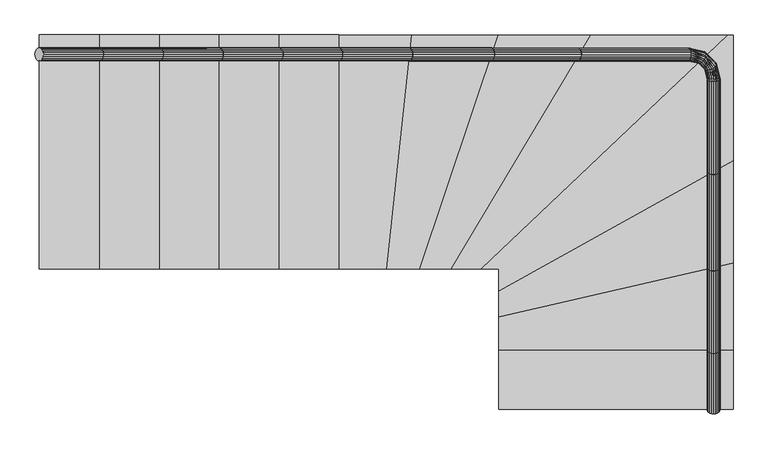
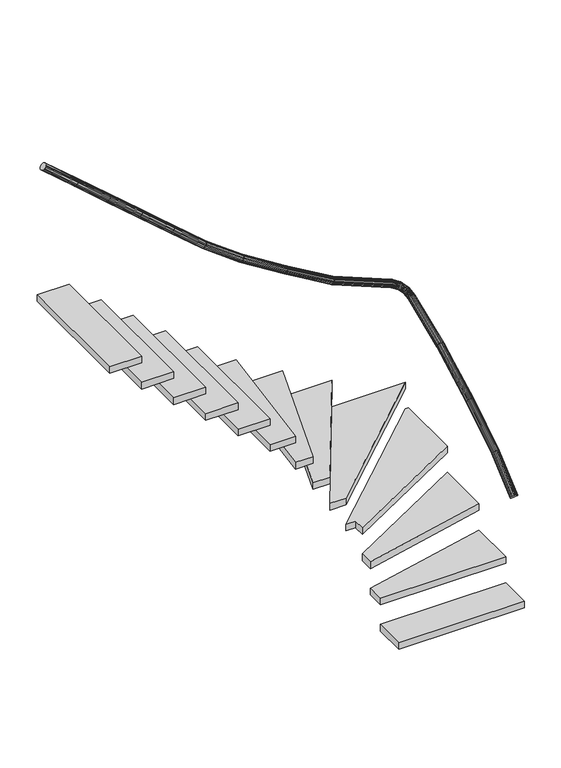
"""IFC4 building model written with IfcOpenShell, lengths in millimetres: stair geometry, 0_3d."""

import ifcopenshell
import ifcopenshell.guid

model = None  # the IFC model being written
_history = None  # IfcOwnerHistory: only IFC2X3 demands one
_inside = {}  # id of a spatial element -> (the spatial element, [elements in it])
_under = {}  # id of a project, library or spatial element -> (it, [spatial elements below it])
_declared = {}  # id of a project -> (the project, [libraries it declares])
_typed = {}  # id of a type object -> (the type object, [elements of that type])
_made_of = {}  # id of a material, layer set ... -> (it, [elements and type objects made of it])


def new_model(schema):
    """Start an empty IFC model of exactly this schema.

    Asked for "IFC4X3", IfcOpenShell would pick the latest addendum, in which some entities
    have other attributes; the version numbers below select the first issue.
    IFC2X3 requires an IfcOwnerHistory on every rooted entity: one is made here for all.
    """
    global model, _history
    if schema == "IFC4X3":
        model = ifcopenshell.file(schema_version=(4, 3, 0, 0))
    else:
        model = ifcopenshell.file(schema=schema)
    _inside.clear()
    _under.clear()
    _declared.clear()
    _typed.clear()
    _made_of.clear()
    _history = None
    if model.schema == "IFC2X3":
        org = make("IfcOrganization", Name="unknown")
        user = make(
            "IfcPersonAndOrganization",
            ThePerson=make("IfcPerson", FamilyName="unknown"),
            TheOrganization=org,
        )
        app = make(
            "IfcApplication",
            ApplicationDeveloper=org,
            Version="unknown",
            ApplicationFullName="unknown",
            ApplicationIdentifier="unknown",
        )
        _history = make(
            "IfcOwnerHistory",
            OwningUser=user,
            OwningApplication=app,
            ChangeAction="ADDED",
            CreationDate=0,
        )
    return model


def make(cls, **values):
    """One entity of the class cls with the attributes given. An attribute that is None is left unset."""
    return model.create_entity(
        cls, **{name: value for name, value in values.items() if value is not None}
    )


def rooted(cls, **values):
    """An entity with a GlobalId (a new one), such as an element, a storey or a relation."""
    return make(cls, GlobalId=ifcopenshell.guid.new(), OwnerHistory=_history, **values)


def si_unit(unit_type, name, prefix=None):
    """IfcSIUnit, for example si_unit("LENGTHUNIT", "METRE", prefix="MILLI")."""
    return make("IfcSIUnit", UnitType=unit_type, Prefix=prefix, Name=name)


def assignment(units):
    """IfcUnitAssignment: the units of a project."""
    return None if units is None else make("IfcUnitAssignment", Units=units)


def point(xyz):
    """IfcCartesianPoint."""
    return None if xyz is None else make("IfcCartesianPoint", Coordinates=xyz)


def direction(xyz):
    """IfcDirection."""
    return None if xyz is None else make("IfcDirection", DirectionRatios=xyz)


def frame(location, z_axis=None, x_axis=None):
    """IfcAxis2Placement3D, a coordinate frame: its origin and axes. An axis left out is left unset."""
    return make(
        "IfcAxis2Placement3D",
        Location=point(location),
        Axis=direction(z_axis),
        RefDirection=direction(x_axis),
    )


def origin():
    """The frame at (0, 0, 0) with its axes left unset."""
    return frame((0.0, 0.0, 0.0))


def origin_with_axes():
    """The frame at (0, 0, 0) with the z axis (0, 0, 1) and the x axis (1, 0, 0) written out."""
    return frame((0.0, 0.0, 0.0), z_axis=(0.0, 0.0, 1.0), x_axis=(1.0, 0.0, 0.0))


def place(relative_to, where):
    """IfcLocalPlacement: puts the frame where relative to a parent placement (None: the world)."""
    return make(
        "IfcLocalPlacement", PlacementRelTo=relative_to, RelativePlacement=where
    )


def context(
    kind, dimensions, precision=None, world=None, true_north=None, identifier=None
):
    """IfcGeometricRepresentationContext, for example the 3D "Model" context."""
    return make(
        "IfcGeometricRepresentationContext",
        ContextIdentifier=identifier,
        ContextType=kind,
        CoordinateSpaceDimension=dimensions,
        Precision=precision,
        WorldCoordinateSystem=world,
        TrueNorth=true_north,
    )


def project(units=None, contexts=None):
    """IfcProject with its units and contexts."""
    return rooted(
        "IfcProject",
        Name="project",
        RepresentationContexts=contexts,
        UnitsInContext=assignment(units),
    )


def spatial(cls, under=None, at=None, **own):
    """A site, building, storey or space (cls), placed at a placement, below another one or the project."""
    s = rooted(cls, ObjectPlacement=at, **own)
    if under is not None:
        _under.setdefault(under.id(), (under, []))[1].append(s)
    return s


def polyline(points):
    """IfcPolyline through the points."""
    return make("IfcPolyline", Points=[point(p) for p in points])


def outline(outer, holes=None, kind="AREA"):
    """IfcArbitraryClosedProfileDef: a profile drawn as a closed curve; with holes, ...WithVoids."""
    if holes is None:
        return make("IfcArbitraryClosedProfileDef", ProfileType=kind, OuterCurve=outer)
    return make(
        "IfcArbitraryProfileDefWithVoids",
        ProfileType=kind,
        OuterCurve=outer,
        InnerCurves=holes,
    )


def extrude(swept, where, along, depth):
    """IfcExtrudedAreaSolid: the profile swept, set in the frame where, extruded along a direction by depth."""
    return make(
        "IfcExtrudedAreaSolid",
        SweptArea=swept,
        Position=where,
        ExtrudedDirection=direction(along),
        Depth=depth,
    )


def faces_of(points, faces, orient=None, outer=None):
    """IfcFace entities. A face is a list of loops; a loop is a list of indices into points, from 0.

    orient and outer hold one flag for each loop. By default every Orientation is true, the
    first loop of a face is its IfcFaceOuterBound and the others are IfcFaceBound.
    """
    made = []
    for i, loops in enumerate(faces):
        bounds = []
        for j, loop in enumerate(loops):
            is_outer = j == 0 if outer is None else outer[i][j]
            bounds.append(
                make(
                    "IfcFaceOuterBound" if is_outer else "IfcFaceBound",
                    Bound=make("IfcPolyLoop", Polygon=[points[k] for k in loop]),
                    Orientation=True if orient is None else orient[i][j],
                )
            )
        made.append(make("IfcFace", Bounds=bounds))
    return made


def faceted_brep(points, faces, orient=None, outer=None, voids=None):
    """IfcFacetedBrep: a solid bounded by flat faces; with voids (closed shells), ...WithVoids."""
    shared = [point(p) for p in points]
    hull = make("IfcClosedShell", CfsFaces=faces_of(shared, faces, orient, outer))
    if voids is None:
        return make("IfcFacetedBrep", Outer=hull)
    return make(
        "IfcFacetedBrepWithVoids",
        Outer=hull,
        Voids=[
            make(cls, CfsFaces=faces_of(shared, fs, o, b)) for cls, fs, o, b in voids
        ],
    )


def shape(context_of_items, identifier, shape_type, items):
    """IfcShapeRepresentation: the items that make up one representation, for example the "Body"."""
    return make(
        "IfcShapeRepresentation",
        ContextOfItems=context_of_items,
        RepresentationIdentifier=identifier,
        RepresentationType=shape_type,
        Items=items,
    )


def source(mapping_origin, context_of_items, identifier, shape_type, items):
    """IfcRepresentationMap: a shape defined once, which mapped items show again and again."""
    return make(
        "IfcRepresentationMap",
        MappingOrigin=mapping_origin,
        MappedRepresentation=shape(context_of_items, identifier, shape_type, items),
    )


def transform(
    local_origin,
    x_axis=None,
    y_axis=None,
    z_axis=None,
    scale=None,
    scale2=None,
    scale3=None,
    uniform=True,
):
    """IfcCartesianTransformationOperator3D, or its non-uniform kind. x_axis, y_axis, z_axis: its Axis1, 2, 3."""
    if uniform:
        return make(
            "IfcCartesianTransformationOperator3D",
            Axis1=direction(x_axis),
            Axis2=direction(y_axis),
            LocalOrigin=point(local_origin),
            Scale=scale,
            Axis3=direction(z_axis),
        )
    return make(
        "IfcCartesianTransformationOperator3DnonUniform",
        Axis1=direction(x_axis),
        Axis2=direction(y_axis),
        LocalOrigin=point(local_origin),
        Scale=scale,
        Axis3=direction(z_axis),
        Scale2=scale2,
        Scale3=scale3,
    )


def mapped(mapping_source, mapping_target):
    """IfcMappedItem: shows the shape of a source again, moved by a transform."""
    return make(
        "IfcMappedItem", MappingSource=mapping_source, MappingTarget=mapping_target
    )


def made_of(thing, what):
    """Note that an element or type object is made of a material, layer set ...; save() writes the relation."""
    if what is not None:
        _made_of.setdefault(what.id(), (what, []))[1].append(thing)
    return thing


def element(
    cls,
    number,
    at=None,
    inside=None,
    cuts=None,
    type_object=None,
    material=None,
    context=None,
    identifier="Body",
    shape_type=None,
    held_by="IfcProductDefinitionShape",
    body=None,
    shapes=None,
    **own,
):
    """One element of the class cls, such as IfcWall. Its Tag is "e" and its number.

    at: its placement. inside: the storey or other place that contains it. cuts: it is an
    opening in that element (IfcRelVoidsElement). A single representation is given by context,
    identifier, shape_type and body (its items); several are given by shapes. held_by: the class
    of the entity that holds the representations. save() writes the other relations.
    """
    e = rooted(cls, Tag="e%d" % number, ObjectPlacement=at, **own)
    if body is not None:
        shapes = [shape(context, identifier, shape_type, body)]
    if shapes is not None:
        e.Representation = make(held_by, Representations=shapes)
    if inside is not None:
        _inside.setdefault(inside.id(), (inside, []))[1].append(e)
    if cuts is not None:
        rooted(
            "IfcRelVoidsElement", RelatingBuildingElement=cuts, RelatedOpeningElement=e
        )
    if type_object is not None:
        _typed.setdefault(type_object.id(), (type_object, []))[1].append(e)
    return made_of(e, material)


def aggregate(whole, parts):
    """IfcRelAggregates: a whole, such as a stair, and the parts it consists of."""
    return rooted("IfcRelAggregates", RelatingObject=whole, RelatedObjects=parts)


def save(model, path):
    """Write the relations noted so far, then the file.

    IfcRelAggregates (storeys below a building ...), IfcRelContainedInSpatialStructure (elements
    in a storey), IfcRelDefinesByType, IfcRelAssociatesMaterial and IfcRelDeclares: one each for
    every whole, place, type object, material and project.
    """
    for whole, parts in _under.values():
        aggregate(whole, parts)
    for where, things in _inside.values():
        rooted(
            "IfcRelContainedInSpatialStructure",
            RelatedElements=things,
            RelatingStructure=where,
        )
    for kind, things in _typed.values():
        rooted("IfcRelDefinesByType", RelatedObjects=things, RelatingType=kind)
    for what, things in _made_of.values():
        rooted("IfcRelAssociatesMaterial", RelatedObjects=things, RelatingMaterial=what)
    for by, libraries in _declared.values():
        rooted("IfcRelDeclares", RelatingContext=by, RelatedDefinitions=libraries)
    model.write(path)


def stair_9e6d9002(model_context):
    return source(origin(), model_context, "Body", "SolidModel", [
        extrude(outline(polyline([(1781.5036957, 473.824936), (1781.5036957, 556.9018591), (1711.5036957, 556.9018591), (2658.8332796, 1456.9018591), (2681.5036957, 1456.9018591), (2681.5036957, 973.1970565), (1781.5036957, 473.824936)])), frame((0.0, 0.0, 595.7142857), z_axis=(0.0, 0.0, 1.0), x_axis=(1.0, 0.0, 0.0)), (0.0, 0.0, 1.0), 50.0),
        extrude(outline(polyline([(936.9018591, 556.9018591), (706.9018591, 556.9018591), (706.9018591, 1456.9018591), (936.9018591, 1456.9018591), (936.9018591, 556.9018591)])), frame((0.0, 0.0, 1787.1428571), z_axis=(0.0, 0.0, 1.0), x_axis=(1.0, 0.0, 0.0)), (0.0, 0.0, 1.0), 50.0),
        extrude(outline(polyline([(1.2235871, -7.9923214), (0.0, 0.0), (1.2235871, 7.9923214), (4.7745751, 15.2022987), (10.3053687, 20.9241691), (17.2745751, 24.597836), (25.0, 25.8636953), (32.7254248, 24.597836), (39.6946313, 20.9241691), (45.2254248, 15.2022987), (48.7764129, 7.9923214), (50.0, 0.0), (48.7764129, -7.9923214), (45.2254248, -15.2022986), (39.6946313, -20.9241689), (32.7254248, -24.5978359), (25.0, -25.8636953), (17.2745751, -24.5978359), (10.3053687, -20.9241689), (4.7745751, -15.2022986), (1.2235871, -7.9923214)])), frame((936.9018591, 1406.9018591, 2656.7020937), z_axis=(-0.7569287102857389, 0.0, 0.6534974579485127), x_axis=(0.0, -1.0, 0.0)), (0.0, 0.0, 1.0), 303.8595272),
        extrude(outline(polyline([(1349.1921789, 556.9018591), (1166.9018591, 556.9018591), (1166.9018591, 1456.9018591), (1444.6115394, 1456.9018591), (1349.1921789, 556.9018591)])), frame((0.0, 0.0, 1390.0), z_axis=(0.0, 0.0, 1.0), x_axis=(1.0, 0.0, 0.0)), (0.0, 0.0, 1.0), 50.0),
        extrude(outline(polyline([(1477.0220692, 556.9018591), (1349.1921789, 556.9018591), (1444.6115394, 1456.9018591), (1776.781649, 1456.9018591), (1477.0220692, 556.9018591)])), frame((0.0, 0.0, 1191.4285714), z_axis=(0.0, 0.0, 1.0), x_axis=(1.0, 0.0, 0.0)), (0.0, 0.0, 1.0), 50.0),
        extrude(outline(polyline([(1711.5036957, 556.9018591), (1597.1723093, 556.9018591), (2132.6233472, 1456.9018591), (2658.8332796, 1456.9018591), (1711.5036957, 556.9018591)])), frame((0.0, 0.0, 794.2857143), z_axis=(0.0, 0.0, 1.0), x_axis=(1.0, 0.0, 0.0)), (0.0, 0.0, 1.0), 50.0),
        extrude(outline(polyline([(1.2235871, -7.9923214), (0.0, 0.0), (1.2235871, 7.9923214), (4.7745751, 15.2022986), (10.3053687, 20.924169), (17.2745751, 24.5978359), (25.0, 25.8636953), (32.7254248, 24.5978359), (39.6946313, 20.924169), (45.2254248, 15.2022986), (48.7764129, 7.9923214), (50.0, 0.0), (48.7764129, -7.9923214), (45.2254248, -15.2022986), (39.6946313, -20.924169), (32.7254248, -24.597836), (25.0, -25.8636953), (17.2745751, -24.597836), (10.3053687, -20.924169), (4.7745751, -15.2022986), (1.2235871, -7.9923214)])), frame((246.9018591, 1406.9018591, 3252.4163795), z_axis=(-0.7569287102857456, 0.0, 0.6534974579485049), x_axis=(0.0, -1.0, 0.0)), (0.0, 0.0, 1.0), 303.8595272),
        faceted_brep([(2630.2801086, 935.0213576, 1458.0478269), (2631.5036957, 931.5827131, 1465.2735223), (2630.2801086, 928.1440687, 1472.4992177), (2626.7291206, 925.0420228, 1479.0176117), (2621.198327, 922.5802252, 1484.1906384), (2614.2291206, 920.9996538, 1487.511926), (2606.5036957, 920.4550261, 1488.6563638), (2598.7782709, 920.9996538, 1487.511926), (2591.8090644, 922.5802252, 1484.1906384), (2586.2782709, 925.0420228, 1479.0176117), (2582.7272828, 928.1440687, 1472.4992177), (2581.5036957, 931.5827131, 1465.2735223), (2582.7272828, 935.0213576, 1458.0478269), (2586.2782709, 938.1234035, 1451.529433), (2591.8090644, 940.5852011, 1446.3564062), (2598.7782709, 942.1657724, 1443.0351186), (2606.5036957, 942.7104002, 1441.8906809), (2614.2291206, 942.1657724, 1443.0351186), (2621.198327, 940.5852011, 1446.3564062), (2626.7291206, 938.1234035, 1451.529433), (2630.2801086, 1283.3224302, 1620.3777918), (2631.5036957, 1286.3944101, 1612.9994356), (2630.2801086, 1289.46639, 1605.6210794), (2626.7291206, 1292.2376632, 1598.9649681), (2621.198327, 1294.436958, 1593.6826483), (2614.2291206, 1295.8489921, 1590.2911902), (2606.5036957, 1296.335546, 1589.1225734), (2598.7782709, 1295.8489921, 1590.2911902), (2591.8090644, 1294.436958, 1593.6826483), (2586.2782709, 1292.2376632, 1598.9649681), (2582.7272828, 1289.46639, 1605.6210794), (2581.5036957, 1286.3944101, 1612.9994356), (2582.7272828, 1283.3224302, 1620.3777918), (2586.2782709, 1280.5511571, 1627.0339031), (2591.8090644, 1278.3518623, 1632.3162229), (2598.7782709, 1276.9398281, 1635.707681), (2606.5036957, 1276.4532743, 1636.8762979), (2614.2291206, 1276.9398281, 1635.707681), (2621.198327, 1278.3518623, 1632.3162229), (2626.7291206, 1280.5511571, 1627.0339031)], [[[0, 1, 2, 3, 4, 5, 6, 7, 8, 9, 10, 11, 12, 13, 14, 15, 16, 17, 18, 19]], [[20, 21, 22, 23, 24, 25, 26, 27, 28, 29, 30, 31, 32, 33, 34, 35, 36, 37, 38, 39]], [[2, 1, 21, 20]], [[3, 2, 20, 39]], [[4, 3, 39, 38]], [[5, 4, 38, 37]], [[6, 5, 37, 36]], [[7, 6, 36, 35]], [[8, 7, 35, 34]], [[9, 8, 34, 33]], [[10, 9, 33, 32]], [[11, 10, 32, 31]], [[12, 11, 31, 30]], [[13, 12, 30, 29]], [[14, 13, 29, 28]], [[15, 14, 28, 27]], [[16, 15, 27, 26]], [[17, 16, 26, 25]], [[18, 17, 25, 24]], [[19, 18, 24, 23]], [[0, 19, 23, 22]], [[1, 0, 22, 21]]]),
        extrude(outline(polyline([(1781.5036957, 373.9346688), (1781.5036957, 473.824936), (2681.5036957, 973.1970565), (2681.5036957, 579.8690495), (1781.5036957, 373.9346688)])), frame((0.0, 0.0, 397.1428571), z_axis=(0.0, 0.0, 1.0), x_axis=(1.0, 0.0, 0.0)), (0.0, 0.0, 1.0), 50.0),
        extrude(outline(polyline([(1.2235871, -7.9923214), (0.0, 0.0), (1.2235871, 7.9923214), (4.7745751, 15.2022986), (10.3053687, 20.9241691), (17.2745751, 24.5978359), (25.0, 25.8636953), (32.7254248, 24.5978359), (39.6946313, 20.9241691), (45.2254248, 15.2022986), (48.7764129, 7.9923214), (50.0, 0.0), (48.7764129, -7.9923214), (45.2254248, -15.2022986), (39.6946313, -20.924169), (32.7254248, -24.5978359), (25.0, -25.8636953), (17.2745751, -24.5978359), (10.3053687, -20.924169), (4.7745751, -15.2022986), (1.2235871, -7.9923214)])), frame((476.9018591, 1406.9018591, 3053.8449509), z_axis=(-0.7569287102857636, 0.0, 0.6534974579484839), x_axis=(0.0, -1.0, 0.0)), (0.0, 0.0, 1.0), 303.8595272),
        faceted_brep([(2630.2801086, 566.7337566, 1259.7925307), (2631.5036957, 562.7078511, 1266.7020937), (2630.2801086, 558.6819455, 1273.6116568), (2626.7291206, 555.0501237, 1279.8448636), (2621.198327, 552.1678935, 1284.7915646), (2614.2291206, 550.3173878, 1287.9675421), (2606.5036957, 549.679747, 1289.0619094), (2598.7782709, 550.3173878, 1287.9675421), (2591.8090644, 552.1678935, 1284.7915646), (2586.2782709, 555.0501237, 1279.8448636), (2582.7272828, 558.6819455, 1273.6116568), (2581.5036957, 562.7078511, 1266.7020937), (2582.7272828, 566.7337566, 1259.7925307), (2586.2782709, 570.3655785, 1253.5593239), (2591.8090644, 573.2478087, 1248.6126229), (2598.7782709, 575.0983143, 1245.4366454), (2606.5036957, 575.7359551, 1244.3422781), (2614.2291206, 575.0983143, 1245.4366454), (2621.198327, 573.2478087, 1248.6126229), (2626.7291206, 570.3655785, 1253.5593239), (2630.2801086, 928.1440687, 1472.4992177), (2631.5036957, 931.5827131, 1465.2735223), (2630.2801086, 935.0213576, 1458.0478269), (2626.7291206, 938.1234035, 1451.529433), (2621.198327, 940.5852011, 1446.3564062), (2614.2291206, 942.1657724, 1443.0351186), (2606.5036957, 942.7104002, 1441.8906809), (2598.7782709, 942.1657724, 1443.0351186), (2591.8090644, 940.5852011, 1446.3564062), (2586.2782709, 938.1234035, 1451.529433), (2582.7272828, 935.0213576, 1458.0478269), (2581.5036957, 931.5827131, 1465.2735223), (2582.7272828, 928.1440687, 1472.4992177), (2586.2782709, 925.0420228, 1479.0176117), (2591.8090644, 922.5802252, 1484.1906384), (2598.7782709, 920.9996538, 1487.511926), (2606.5036957, 920.4550261, 1488.6563638), (2614.2291206, 920.9996538, 1487.511926), (2621.198327, 922.5802252, 1484.1906384), (2626.7291206, 925.0420228, 1479.0176117)], [[[0, 1, 2, 3, 4, 5, 6, 7, 8, 9, 10, 11, 12, 13, 14, 15, 16, 17, 18, 19]], [[20, 21, 22, 23, 24, 25, 26, 27, 28, 29, 30, 31, 32, 33, 34, 35, 36, 37, 38, 39]], [[2, 1, 21, 20]], [[3, 2, 20, 39]], [[4, 3, 39, 38]], [[5, 4, 38, 37]], [[6, 5, 37, 36]], [[7, 6, 36, 35]], [[8, 7, 35, 34]], [[9, 8, 34, 33]], [[10, 9, 33, 32]], [[11, 10, 32, 31]], [[12, 11, 31, 30]], [[13, 12, 30, 29]], [[14, 13, 29, 28]], [[15, 14, 28, 27]], [[16, 15, 27, 26]], [[17, 16, 26, 25]], [[18, 17, 25, 24]], [[19, 18, 24, 23]], [[0, 19, 23, 22]], [[1, 0, 22, 21]]]),
        faceted_brep([(2630.2801086, 251.6675536, 1061.6862641), (2631.5036957, 246.9018591, 1068.1306652), (2630.2801086, 242.1361647, 1074.5750662), (2626.7291206, 237.8369696, 1080.3886444), (2621.198327, 234.4251091, 1085.0023262), (2614.2291206, 232.2345598, 1087.9644922), (2606.5036957, 231.4797479, 1088.985185), (2598.7782709, 232.2345598, 1087.9644922), (2591.8090644, 234.4251091, 1085.0023262), (2586.2782709, 237.8369696, 1080.3886444), (2582.7272828, 242.1361647, 1074.5750662), (2581.5036957, 246.9018591, 1068.1306652), (2582.7272828, 251.6675536, 1061.6862641), (2586.2782709, 255.9667486, 1055.872686), (2591.8090644, 259.3786091, 1051.2590042), (2598.7782709, 261.5691584, 1048.2968382), (2606.5036957, 262.3239703, 1047.2761453), (2614.2291206, 261.5691584, 1048.2968382), (2621.198327, 259.3786091, 1051.2590042), (2626.7291206, 255.9667486, 1055.872686), (2630.2801086, 558.6819455, 1273.6116568), (2631.5036957, 562.7078511, 1266.7020937), (2630.2801086, 566.7337566, 1259.7925307), (2626.7291206, 570.3655785, 1253.5593239), (2621.198327, 573.2478087, 1248.6126229), (2614.2291206, 575.0983143, 1245.4366454), (2606.5036957, 575.7359551, 1244.3422781), (2598.7782709, 575.0983143, 1245.4366454), (2591.8090644, 573.2478087, 1248.6126229), (2586.2782709, 570.3655785, 1253.5593239), (2582.7272828, 566.7337566, 1259.7925307), (2581.5036957, 562.7078511, 1266.7020937), (2582.7272828, 558.6819455, 1273.6116568), (2586.2782709, 555.0501237, 1279.8448636), (2591.8090644, 552.1678935, 1284.7915646), (2598.7782709, 550.3173878, 1287.9675421), (2606.5036957, 549.679747, 1289.0619094), (2614.2291206, 550.3173878, 1287.9675421), (2621.198327, 552.1678935, 1284.7915646), (2626.7291206, 555.0501237, 1279.8448636)], [[[0, 1, 2, 3, 4, 5, 6, 7, 8, 9, 10, 11, 12, 13, 14, 15, 16, 17, 18, 19]], [[20, 21, 22, 23, 24, 25, 26, 27, 28, 29, 30, 31, 32, 33, 34, 35, 36, 37, 38, 39]], [[2, 1, 21, 20]], [[3, 2, 20, 39]], [[4, 3, 39, 38]], [[5, 4, 38, 37]], [[6, 5, 37, 36]], [[7, 6, 36, 35]], [[8, 7, 35, 34]], [[9, 8, 34, 33]], [[10, 9, 33, 32]], [[11, 10, 32, 31]], [[12, 11, 31, 30]], [[13, 12, 30, 29]], [[14, 13, 29, 28]], [[15, 14, 28, 27]], [[16, 15, 27, 26]], [[17, 16, 26, 25]], [[18, 17, 25, 24]], [[19, 18, 24, 23]], [[0, 19, 23, 22]], [[1, 0, 22, 21]]]),
        faceted_brep([(2630.2801086, 1289.46639, 1605.6210794), (2631.5036957, 1286.3944101, 1612.9994356), (2630.2801086, 1283.3224302, 1620.3777918), (2626.7291206, 1280.5511571, 1627.0339031), (2621.198327, 1278.3518623, 1632.3162229), (2614.2291206, 1276.9398281, 1635.707681), (2606.5036957, 1276.4532743, 1636.8762979), (2598.7782709, 1276.9398281, 1635.707681), (2591.8090644, 1278.3518623, 1632.3162229), (2586.2782709, 1280.5511571, 1627.0339031), (2582.7272828, 1283.3224302, 1620.3777918), (2581.5036957, 1286.3944101, 1612.9994356), (2582.7272828, 1289.46639, 1605.6210794), (2586.2782709, 1292.2376632, 1598.9649681), (2591.8090644, 1294.436958, 1593.6826483), (2598.7782709, 1295.8489921, 1590.2911902), (2606.5036957, 1296.335546, 1589.1225734), (2614.2291206, 1295.8489921, 1590.2911902), (2621.198327, 1294.436958, 1593.6826483), (2626.7291206, 1292.2376632, 1598.9649681), (2616.4980036, 1348.8501513, 1638.9123688), (2617.3046378, 1344.8271855, 1645.879395), (2615.8855438, 1340.0232633, 1652.1644401), (2612.3796323, 1334.9086261, 1657.1522801), (2607.1300863, 1329.9839302, 1660.3546705), (2600.650768, 1325.7312391, 1661.4581391), (2593.5759183, 1322.5668359, 1660.3546705), (2586.5980727, 1320.8004745, 1657.1522801), (2580.4002713, 1320.6050585, 1652.1644401), (2575.5891981, 1321.9997167, 1645.879395), (2572.6357946, 1324.8479302, 1638.9123688), (2571.8291603, 1328.870896, 1631.9453426), (2573.2482544, 1333.6748181, 1625.6602975), (2576.7541659, 1338.7894554, 1620.6724574), (2582.0037118, 1343.7141513, 1617.470067), (2588.4830301, 1347.9668423, 1616.3665985), (2595.5578799, 1351.1312455, 1617.470067), (2602.5357255, 1352.8976069, 1620.6724574), (2608.7335269, 1353.0930229, 1625.6602975), (2613.5446, 1351.6983647, 1631.9453426), (2573.2894856, 1391.9456089, 1666.2859781), (2576.1190741, 1389.0124344, 1673.2691208), (2577.5017941, 1384.2169558, 1679.5687049), (2577.3022952, 1378.028588, 1684.5680831), (2575.5401057, 1371.0530916, 1687.7778814), (2572.3877211, 1363.9732768, 1688.8839026), (2568.1537188, 1357.4821652, 1687.7778814), (2563.2525523, 1352.215152, 1684.5680831), (2558.163982, 1348.6878091, 1679.5687049), (2553.3861126, 1347.2454175, 1673.2691208), (2549.3866353, 1348.0291684, 1666.2859781), (2546.5570467, 1350.962343, 1659.3028354), (2545.1743267, 1355.7578216, 1653.0032514), (2545.3738257, 1361.9461894, 1648.0038732), (2547.1360151, 1368.9216857, 1644.7940748), (2550.2883997, 1376.0015006, 1643.6880537), (2554.5224021, 1382.4926122, 1644.7940748), (2559.4235686, 1387.7596254, 1648.0038732), (2564.5121389, 1391.2869683, 1653.0032514), (2569.2900082, 1392.7293599, 1659.3028354), (2510.6895066, 1406.9018591, 1691.7803901), (2513.6813624, 1405.678272, 1699.1915978), (2516.3803544, 1402.127284, 1705.8773449), (2518.5222867, 1396.5964904, 1711.1831838), (2519.8974918, 1389.627284, 1714.5897421), (2520.3713552, 1381.9018591, 1715.7635621), (2519.8974918, 1374.1764343, 1714.5897421), (2518.5222867, 1367.2072278, 1711.1831838), (2516.3803544, 1361.6764343, 1705.8773449), (2513.6813624, 1358.1254462, 1699.1915978), (2510.6895066, 1356.9018591, 1691.7803901), (2507.6976509, 1358.1254462, 1684.3691823), (2504.9986588, 1361.6764343, 1677.6834352), (2502.8567266, 1367.2072278, 1672.3775963), (2501.4815215, 1374.1764343, 1668.971038), (2501.0076581, 1381.9018591, 1667.797218), (2501.4815215, 1389.627284, 1668.971038), (2502.8567266, 1396.5964904, 1672.3775963), (2504.9986588, 1402.127284, 1677.6834352), (2507.6976509, 1405.678272, 1684.3691823), (2091.5504886, 1405.678272, 1869.6030507), (2088.0024274, 1406.9018591, 1862.4163795), (2084.4543661, 1405.678272, 1855.2297082), (2081.2536138, 1402.127284, 1848.7465184), (2078.7134824, 1396.5964904, 1843.6014299), (2077.0826177, 1389.627284, 1840.2980797), (2076.52066, 1381.9018591, 1839.1598228), (2077.0826177, 1374.1764343, 1840.2980797), (2078.7134824, 1367.2072278, 1843.6014299), (2081.2536138, 1361.6764343, 1848.7465184), (2084.4543661, 1358.1254462, 1855.2297082), (2088.0024274, 1356.9018591, 1862.4163795), (2091.5504886, 1358.1254462, 1869.6030507), (2094.7512409, 1361.6764343, 1876.0862405), (2097.2913723, 1367.2072278, 1881.231329), (2098.9222371, 1374.1764343, 1884.5346792), (2099.4841948, 1381.9018591, 1885.6729361), (2098.9222371, 1389.627284, 1884.5346792), (2097.2913723, 1396.5964904, 1881.231329), (2094.7512409, 1402.127284, 1876.0862405)], [[[0, 1, 2, 3, 4, 5, 6, 7, 8, 9, 10, 11, 12, 13, 14, 15, 16, 17, 18, 19]], [[2, 1, 20]], [[21, 2, 20]], [[3, 2, 21]], [[22, 3, 21]], [[4, 3, 22]], [[23, 4, 22]], [[5, 4, 23]], [[24, 5, 23]], [[6, 5, 24]], [[25, 6, 24]], [[7, 6, 25]], [[26, 7, 25]], [[8, 7, 26]], [[27, 8, 26]], [[9, 8, 27]], [[28, 9, 27]], [[10, 9, 28]], [[29, 10, 28]], [[11, 10, 29]], [[30, 11, 29]], [[12, 11, 30]], [[31, 12, 30]], [[13, 12, 31]], [[32, 13, 31]], [[14, 13, 32]], [[33, 14, 32]], [[15, 14, 33]], [[34, 15, 33]], [[16, 15, 34]], [[35, 16, 34]], [[17, 16, 35]], [[36, 17, 35]], [[18, 17, 36]], [[37, 18, 36]], [[19, 18, 37]], [[38, 19, 37]], [[0, 19, 38]], [[39, 0, 38]], [[1, 0, 39]], [[20, 1, 39]], [[21, 20, 40]], [[41, 21, 40]], [[22, 21, 41]], [[42, 22, 41]], [[23, 22, 42]], [[43, 23, 42]], [[24, 23, 43]], [[44, 24, 43]], [[25, 24, 44]], [[45, 25, 44]], [[26, 25, 45]], [[46, 26, 45]], [[27, 26, 46]], [[47, 27, 46]], [[28, 27, 47]], [[48, 28, 47]], [[29, 28, 48]], [[49, 29, 48]], [[30, 29, 49]], [[50, 30, 49]], [[31, 30, 50]], [[51, 31, 50]], [[32, 31, 51]], [[52, 32, 51]], [[33, 32, 52]], [[53, 33, 52]], [[34, 33, 53]], [[54, 34, 53]], [[35, 34, 54]], [[55, 35, 54]], [[36, 35, 55]], [[56, 36, 55]], [[37, 36, 56]], [[57, 37, 56]], [[38, 37, 57]], [[58, 38, 57]], [[39, 38, 58]], [[59, 39, 58]], [[20, 39, 59]], [[40, 20, 59]], [[41, 40, 60]], [[61, 41, 60]], [[42, 41, 61]], [[62, 42, 61]], [[43, 42, 62]], [[63, 43, 62]], [[44, 43, 63]], [[64, 44, 63]], [[45, 44, 64]], [[65, 45, 64]], [[46, 45, 65]], [[66, 46, 65]], [[47, 46, 66]], [[67, 47, 66]], [[48, 47, 67]], [[68, 48, 67]], [[49, 48, 68]], [[69, 49, 68]], [[50, 49, 69]], [[70, 50, 69]], [[51, 50, 70]], [[71, 51, 70]], [[52, 51, 71]], [[72, 52, 71]], [[53, 52, 72]], [[73, 53, 72]], [[54, 53, 73]], [[74, 54, 73]], [[55, 54, 74]], [[75, 55, 74]], [[56, 55, 75]], [[76, 56, 75]], [[57, 56, 76]], [[77, 57, 76]], [[58, 57, 77]], [[78, 58, 77]], [[59, 58, 78]], [[79, 59, 78]], [[40, 59, 79]], [[60, 40, 79]], [[80, 81, 82, 83, 84, 85, 86, 87, 88, 89, 90, 91, 92, 93, 94, 95, 96, 97, 98, 99]], [[61, 60, 81, 80]], [[62, 61, 80, 99]], [[63, 62, 99, 98]], [[64, 63, 98, 97]], [[65, 64, 97, 96]], [[66, 65, 96, 95]], [[67, 66, 95, 94]], [[68, 67, 94, 93]], [[69, 68, 93, 92]], [[70, 69, 92, 91]], [[71, 70, 91, 90]], [[72, 71, 90, 89]], [[73, 72, 89, 88]], [[74, 73, 88, 87]], [[75, 74, 87, 86]], [[76, 75, 86, 85]], [[77, 76, 85, 84]], [[78, 77, 84, 83]], [[79, 78, 83, 82]], [[60, 79, 82, 81]]]),
        extrude(outline(polyline([(1781.5036957, 16.9018591), (1781.5036957, 246.9018591), (2681.5036957, 246.9018591), (2681.5036957, 16.9018591), (1781.5036957, 16.9018591)])), origin_with_axes(), (0.0, 0.0, 1.0), 50.0),
        extrude(outline(polyline([(246.9018591, 556.9018591), (16.9018591, 556.9018591), (16.9018591, 1456.9018591), (246.9018591, 1456.9018591), (246.9018591, 556.9018591)])), frame((0.0, 0.0, 2382.8571429), z_axis=(0.0, 0.0, 1.0), x_axis=(1.0, 0.0, 0.0)), (0.0, 0.0, 1.0), 50.0),
        extrude(outline(polyline([(1.2235871, -7.9923214), (0.0, 0.0), (1.2235871, 7.9923214), (4.7745751, 15.2022986), (10.3053687, 20.9241691), (17.2745751, 24.5978359), (25.0, 25.8636953), (32.7254248, 24.5978359), (39.6946313, 20.9241691), (45.2254248, 15.2022986), (48.7764129, 7.9923214), (50.0, 0.0), (48.7764129, -7.9923214), (45.2254248, -15.2022986), (39.6946313, -20.9241689), (32.7254248, -24.5978359), (25.0, -25.8636953), (17.2745751, -24.5978359), (10.3053687, -20.9241689), (4.7745751, -15.2022986), (1.2235871, -7.9923214)])), frame((706.9018591, 1406.9018591, 2855.2735223), z_axis=(-0.756928710285736, 0.0, 0.6534974579485159), x_axis=(0.0, -1.0, 0.0)), (0.0, 0.0, 1.0), 303.8595272),
        faceted_brep([(1747.6382113, 1405.678272, 2054.1646194), (1751.801684, 1406.9018591, 2060.987808), (1755.9651567, 1405.678272, 2067.8109967), (1759.7210797, 1402.127284, 2073.966284), (1762.701797, 1396.5964904, 2078.8511477), (1764.6155354, 1389.627284, 2081.9874233), (1765.2749647, 1381.9018591, 2083.0681102), (1764.6155354, 1374.1764343, 2081.9874233), (1762.701797, 1367.2072278, 2078.8511477), (1759.7210797, 1361.6764343, 2073.966284), (1755.9651567, 1358.1254462, 2067.8109967), (1751.801684, 1356.9018591, 2060.987808), (1747.6382113, 1358.1254462, 2054.1646194), (1743.8822884, 1361.6764343, 2048.009332), (1740.901571, 1367.2072278, 2043.1244683), (1738.9878327, 1374.1764343, 2039.9881928), (1738.3284034, 1381.9018591, 2038.9075058), (1738.9878327, 1389.627284, 2039.9881928), (1740.901571, 1396.5964904, 2043.1244683), (1743.8822884, 1402.127284, 2048.009332), (1441.1651504, 1405.678272, 2266.1670868), (1436.659926, 1406.9018591, 2259.5592366), (1432.1547015, 1405.678272, 2252.9513864), (1428.0904799, 1402.127284, 2246.9903587), (1424.8650953, 1396.5964904, 2242.2596602), (1422.7942709, 1389.627284, 2239.2223649), (1422.0807134, 1381.9018591, 2238.1757842), (1422.7942709, 1374.1764343, 2239.2223649), (1424.8650953, 1367.2072278, 2242.2596602), (1428.0904799, 1361.6764343, 2246.9903587), (1432.1547015, 1358.1254462, 2252.9513864), (1436.659926, 1356.9018591, 2259.5592366), (1441.1651504, 1358.1254462, 2266.1670868), (1445.2293721, 1361.6764343, 2272.1281145), (1448.4547567, 1367.2072278, 2276.858813), (1450.5255811, 1374.1764343, 2279.8961083), (1451.2391385, 1381.9018591, 2280.942689), (1450.5255811, 1389.627284, 2279.8961083), (1448.4547567, 1396.5964904, 2276.858813), (1445.2293721, 1402.127284, 2272.1281145)], [[[0, 1, 2, 3, 4, 5, 6, 7, 8, 9, 10, 11, 12, 13, 14, 15, 16, 17, 18, 19]], [[20, 21, 22, 23, 24, 25, 26, 27, 28, 29, 30, 31, 32, 33, 34, 35, 36, 37, 38, 39]], [[2, 1, 21, 20]], [[3, 2, 20, 39]], [[4, 3, 39, 38]], [[5, 4, 38, 37]], [[6, 5, 37, 36]], [[7, 6, 36, 35]], [[8, 7, 35, 34]], [[9, 8, 34, 33]], [[10, 9, 33, 32]], [[11, 10, 32, 31]], [[12, 11, 31, 30]], [[13, 12, 30, 29]], [[14, 13, 29, 28]], [[15, 14, 28, 27]], [[16, 15, 27, 26]], [[17, 16, 26, 25]], [[18, 17, 25, 24]], [[19, 18, 24, 23]], [[0, 19, 23, 22]], [[1, 0, 22, 21]]]),
        extrude(outline(polyline([(1597.1723093, 556.9018591), (1477.0220692, 556.9018591), (1776.781649, 1456.9018591), (2132.6233472, 1456.9018591), (1597.1723093, 556.9018591)])), frame((0.0, 0.0, 992.8571429), z_axis=(0.0, 0.0, 1.0), x_axis=(1.0, 0.0, 0.0)), (0.0, 0.0, 1.0), 50.0),
        extrude(outline(polyline([(1166.9018591, 556.9018591), (936.9018591, 556.9018591), (936.9018591, 1456.9018591), (1166.9018591, 1456.9018591), (1166.9018591, 556.9018591)])), frame((0.0, 0.0, 1588.5714286), z_axis=(0.0, 0.0, 1.0), x_axis=(1.0, 0.0, 0.0)), (0.0, 0.0, 1.0), 50.0),
        faceted_brep([(2630.2801086, 22.1248208, 863.5096191), (2631.5036957, 16.9018591, 869.5592366), (2630.2801086, 11.6788974, 875.6088541), (2626.7291206, 6.9671956, 881.0662929), (2621.198327, 3.2279679, 885.3973409), (2614.2291206, 0.8272359, 888.1780448), (2606.5036957, 0.0, 889.1362101), (2598.7782709, 0.8272359, 888.1780448), (2591.8090644, 3.2279679, 885.3973409), (2586.2782709, 6.9671956, 881.0662929), (2582.7272828, 11.6788974, 875.6088541), (2581.5036957, 16.9018591, 869.5592366), (2582.7272828, 22.1248208, 863.5096191), (2586.2782709, 26.8365226, 858.0521803), (2591.8090644, 30.5757504, 853.7211323), (2598.7782709, 32.9764824, 850.9404284), (2606.5036957, 33.8037182, 849.9822631), (2614.2291206, 32.9764824, 850.9404284), (2621.198327, 30.5757504, 853.7211323), (2626.7291206, 26.8365226, 858.0521803), (2630.2801086, 242.1361647, 1074.5750662), (2631.5036957, 246.9018591, 1068.1306652), (2630.2801086, 251.6675536, 1061.6862641), (2626.7291206, 255.9667486, 1055.872686), (2621.198327, 259.3786091, 1051.2590042), (2614.2291206, 261.5691584, 1048.2968382), (2606.5036957, 262.3239703, 1047.2761453), (2598.7782709, 261.5691584, 1048.2968382), (2591.8090644, 259.3786091, 1051.2590042), (2586.2782709, 255.9667486, 1055.872686), (2582.7272828, 251.6675536, 1061.6862641), (2581.5036957, 246.9018591, 1068.1306652), (2582.7272828, 242.1361647, 1074.5750662), (2586.2782709, 237.8369696, 1080.3886444), (2591.8090644, 234.4251091, 1085.0023262), (2598.7782709, 232.2345598, 1087.9644922), (2606.5036957, 231.4797479, 1088.985185), (2614.2291206, 232.2345598, 1087.9644922), (2621.198327, 234.4251091, 1085.0023262), (2626.7291206, 237.8369696, 1080.3886444)], [[[0, 1, 2, 3, 4, 5, 6, 7, 8, 9, 10, 11, 12, 13, 14, 15, 16, 17, 18, 19]], [[20, 21, 22, 23, 24, 25, 26, 27, 28, 29, 30, 31, 32, 33, 34, 35, 36, 37, 38, 39]], [[2, 1, 21, 20]], [[3, 2, 20, 39]], [[4, 3, 39, 38]], [[5, 4, 38, 37]], [[6, 5, 37, 36]], [[7, 6, 36, 35]], [[8, 7, 35, 34]], [[9, 8, 34, 33]], [[10, 9, 33, 32]], [[11, 10, 32, 31]], [[12, 11, 31, 30]], [[13, 12, 30, 29]], [[14, 13, 29, 28]], [[15, 14, 28, 27]], [[16, 15, 27, 26]], [[17, 16, 26, 25]], [[18, 17, 25, 24]], [[19, 18, 24, 23]], [[0, 19, 23, 22]], [[1, 0, 22, 21]]]),
        faceted_brep([(1432.1547015, 1405.678272, 2252.9513864), (1436.659926, 1406.9018591, 2259.5592366), (1441.1651504, 1405.678272, 2266.1670868), (1445.2293721, 1402.127284, 2272.1281145), (1448.4547567, 1396.5964904, 2276.858813), (1450.5255811, 1389.627284, 2279.8961083), (1451.2391385, 1381.9018591, 2280.942689), (1450.5255811, 1374.1764343, 2279.8961083), (1448.4547567, 1367.2072278, 2276.858813), (1445.2293721, 1361.6764343, 2272.1281145), (1441.1651504, 1358.1254462, 2266.1670868), (1436.659926, 1356.9018591, 2259.5592366), (1432.1547015, 1358.1254462, 2252.9513864), (1428.0904799, 1361.6764343, 2246.9903587), (1424.8650953, 1367.2072278, 2242.2596602), (1422.7942709, 1374.1764343, 2239.2223649), (1422.0807134, 1381.9018591, 2238.1757842), (1422.7942709, 1389.627284, 2239.2223649), (1424.8650953, 1396.5964904, 2242.2596602), (1428.0904799, 1402.127284, 2246.9903587), (1171.8898438, 1405.678272, 2464.383151), (1166.9018591, 1406.9018591, 2458.1306652), (1161.9138744, 1405.678272, 2451.8781793), (1157.4141484, 1402.127284, 2446.2377304), (1153.8431456, 1396.5964904, 2441.7614447), (1151.5504206, 1389.627284, 2438.8874925), (1150.7604015, 1381.9018591, 2437.897196), (1151.5504206, 1374.1764343, 2438.8874925), (1153.8431456, 1367.2072278, 2441.7614447), (1157.4141484, 1361.6764343, 2446.2377304), (1161.9138744, 1358.1254462, 2451.8781793), (1166.9018591, 1356.9018591, 2458.1306652), (1171.8898438, 1358.1254462, 2464.383151), (1176.3895699, 1361.6764343, 2470.0236), (1179.9605727, 1367.2072278, 2474.4998856), (1182.2532976, 1374.1764343, 2477.3738379), (1183.0433167, 1381.9018591, 2478.3641344), (1182.2532976, 1389.627284, 2477.3738379), (1179.9605727, 1396.5964904, 2474.4998856), (1176.3895699, 1402.127284, 2470.0236)], [[[0, 1, 2, 3, 4, 5, 6, 7, 8, 9, 10, 11, 12, 13, 14, 15, 16, 17, 18, 19]], [[20, 21, 22, 23, 24, 25, 26, 27, 28, 29, 30, 31, 32, 33, 34, 35, 36, 37, 38, 39]], [[2, 1, 21, 20]], [[3, 2, 20, 39]], [[4, 3, 39, 38]], [[5, 4, 38, 37]], [[6, 5, 37, 36]], [[7, 6, 36, 35]], [[8, 7, 35, 34]], [[9, 8, 34, 33]], [[10, 9, 33, 32]], [[11, 10, 32, 31]], [[12, 11, 31, 30]], [[13, 12, 30, 29]], [[14, 13, 29, 28]], [[15, 14, 28, 27]], [[16, 15, 27, 26]], [[17, 16, 26, 25]], [[18, 17, 25, 24]], [[19, 18, 24, 23]], [[0, 19, 23, 22]], [[1, 0, 22, 21]]]),
        extrude(outline(polyline([(476.9018591, 556.9018591), (246.9018591, 556.9018591), (246.9018591, 1456.9018591), (476.9018591, 1456.9018591), (476.9018591, 556.9018591)])), frame((0.0, 0.0, 2184.2857143), z_axis=(0.0, 0.0, 1.0), x_axis=(1.0, 0.0, 0.0)), (0.0, 0.0, 1.0), 50.0),
        faceted_brep([(2084.4543661, 1405.678272, 1855.2297082), (2088.0024274, 1406.9018591, 1862.4163795), (2091.5504886, 1405.678272, 1869.6030507), (2094.7512409, 1402.127284, 1876.0862405), (2097.2913723, 1396.5964904, 1881.231329), (2098.9222371, 1389.627284, 1884.5346792), (2099.4841948, 1381.9018591, 1885.6729361), (2098.9222371, 1374.1764343, 1884.5346792), (2097.2913723, 1367.2072278, 1881.231329), (2094.7512409, 1361.6764343, 1876.0862405), (2091.5504886, 1358.1254462, 1869.6030507), (2088.0024274, 1356.9018591, 1862.4163795), (2084.4543661, 1358.1254462, 1855.2297082), (2081.2536138, 1361.6764343, 1848.7465184), (2078.7134824, 1367.2072278, 1843.6014299), (2077.0826177, 1374.1764343, 1840.2980797), (2076.52066, 1381.9018591, 1839.1598228), (2077.0826177, 1389.627284, 1840.2980797), (2078.7134824, 1396.5964904, 1843.6014299), (2081.2536138, 1402.127284, 1848.7465184), (1755.9651567, 1405.678272, 2067.8109967), (1751.801684, 1406.9018591, 2060.987808), (1747.6382113, 1405.678272, 2054.1646194), (1743.8822884, 1402.127284, 2048.009332), (1740.901571, 1396.5964904, 2043.1244683), (1738.9878327, 1389.627284, 2039.9881928), (1738.3284034, 1381.9018591, 2038.9075058), (1738.9878327, 1374.1764343, 2039.9881928), (1740.901571, 1367.2072278, 2043.1244683), (1743.8822884, 1361.6764343, 2048.009332), (1747.6382113, 1358.1254462, 2054.1646194), (1751.801684, 1356.9018591, 2060.987808), (1755.9651567, 1358.1254462, 2067.8109967), (1759.7210797, 1361.6764343, 2073.966284), (1762.701797, 1367.2072278, 2078.8511477), (1764.6155354, 1374.1764343, 2081.9874233), (1765.2749647, 1381.9018591, 2083.0681102), (1764.6155354, 1389.627284, 2081.9874233), (1762.701797, 1396.5964904, 2078.8511477), (1759.7210797, 1402.127284, 2073.966284)], [[[0, 1, 2, 3, 4, 5, 6, 7, 8, 9, 10, 11, 12, 13, 14, 15, 16, 17, 18, 19]], [[20, 21, 22, 23, 24, 25, 26, 27, 28, 29, 30, 31, 32, 33, 34, 35, 36, 37, 38, 39]], [[2, 1, 21, 20]], [[3, 2, 20, 39]], [[4, 3, 39, 38]], [[5, 4, 38, 37]], [[6, 5, 37, 36]], [[7, 6, 36, 35]], [[8, 7, 35, 34]], [[9, 8, 34, 33]], [[10, 9, 33, 32]], [[11, 10, 32, 31]], [[12, 11, 31, 30]], [[13, 12, 30, 29]], [[14, 13, 29, 28]], [[15, 14, 28, 27]], [[16, 15, 27, 26]], [[17, 16, 26, 25]], [[18, 17, 25, 24]], [[19, 18, 24, 23]], [[0, 19, 23, 22]], [[1, 0, 22, 21]]]),
        extrude(outline(polyline([(706.9018591, 556.9018591), (476.9018591, 556.9018591), (476.9018591, 1456.9018591), (706.9018591, 1456.9018591), (706.9018591, 556.9018591)])), frame((0.0, 0.0, 1985.7142857), z_axis=(0.0, 0.0, 1.0), x_axis=(1.0, 0.0, 0.0)), (0.0, 0.0, 1.0), 50.0),
        faceted_brep([(1161.9138744, 1405.678272, 2451.8781793), (1166.9018591, 1406.9018591, 2458.1306652), (1171.8898438, 1405.678272, 2464.383151), (1176.3895699, 1402.127284, 2470.0236), (1179.9605727, 1396.5964904, 2474.4998856), (1182.2532976, 1389.627284, 2477.3738379), (1183.0433167, 1381.9018591, 2478.3641344), (1182.2532976, 1374.1764343, 2477.3738379), (1179.9605727, 1367.2072278, 2474.4998856), (1176.3895699, 1361.6764343, 2470.0236), (1171.8898438, 1358.1254462, 2464.383151), (1166.9018591, 1356.9018591, 2458.1306652), (1161.9138744, 1358.1254462, 2451.8781793), (1157.4141484, 1361.6764343, 2446.2377304), (1153.8431456, 1367.2072278, 2441.7614447), (1151.5504206, 1374.1764343, 2438.8874925), (1150.7604015, 1381.9018591, 2437.897196), (1151.5504206, 1389.627284, 2438.8874925), (1153.8431456, 1396.5964904, 2441.7614447), (1157.4141484, 1402.127284, 2446.2377304), (942.1248208, 1405.678272, 2662.7517113), (936.9018591, 1406.9018591, 2656.7020937), (931.6788974, 1405.678272, 2650.6524762), (926.9671956, 1402.127284, 2645.1950374), (923.2279679, 1396.5964904, 2640.8639895), (920.8272359, 1389.627284, 2638.0832855), (920.0, 1381.9018591, 2637.1251202), (920.8272359, 1374.1764343, 2638.0832855), (923.2279679, 1367.2072278, 2640.8639895), (926.9671956, 1361.6764343, 2645.1950374), (931.6788974, 1358.1254462, 2650.6524762), (936.9018591, 1356.9018591, 2656.7020937), (942.1248208, 1358.1254462, 2662.7517113), (946.8365226, 1361.6764343, 2668.2091501), (950.5757504, 1367.2072278, 2672.540198), (952.9764824, 1374.1764343, 2675.320902), (953.8037182, 1381.9018591, 2676.2790673), (952.9764824, 1389.627284, 2675.320902), (950.5757504, 1396.5964904, 2672.540198), (946.8365226, 1402.127284, 2668.2091501)], [[[0, 1, 2, 3, 4, 5, 6, 7, 8, 9, 10, 11, 12, 13, 14, 15, 16, 17, 18, 19]], [[20, 21, 22, 23, 24, 25, 26, 27, 28, 29, 30, 31, 32, 33, 34, 35, 36, 37, 38, 39]], [[2, 1, 21, 20]], [[3, 2, 20, 39]], [[4, 3, 39, 38]], [[5, 4, 38, 37]], [[6, 5, 37, 36]], [[7, 6, 36, 35]], [[8, 7, 35, 34]], [[9, 8, 34, 33]], [[10, 9, 33, 32]], [[11, 10, 32, 31]], [[12, 11, 31, 30]], [[13, 12, 30, 29]], [[14, 13, 29, 28]], [[15, 14, 28, 27]], [[16, 15, 27, 26]], [[17, 16, 26, 25]], [[18, 17, 25, 24]], [[19, 18, 24, 23]], [[0, 19, 23, 22]], [[1, 0, 22, 21]]]),
        extrude(outline(polyline([(1781.5036957, 246.9018591), (1781.5036957, 373.9346688), (2681.5036957, 579.8690495), (2681.5036957, 246.9018591), (1781.5036957, 246.9018591)])), frame((0.0, 0.0, 198.5714286), z_axis=(0.0, 0.0, 1.0), x_axis=(1.0, 0.0, 0.0)), (0.0, 0.0, 1.0), 50.0),
    ])


if __name__ == "__main__":
    model = new_model("IFC4")
    model_context = context("Model", 3, world=origin())
    ifc_project = project(units=[si_unit("LENGTHUNIT", "METRE", prefix="MILLI")], contexts=[model_context])
    site = spatial("IfcSite", under=ifc_project)
    building = spatial("IfcBuilding", under=site)
    placement = place(None, origin())
    stair_shape = stair_9e6d9002(model_context)
    element("IfcStair", 1, ObjectType="0_3d", at=placement, inside=building, context=model_context, shape_type="MappedRepresentation", body=[
        mapped(stair_shape, transform((0.0, 0.0, 0.0), x_axis=(1.0, 0.0, 0.0), y_axis=(0.0, 1.0, 0.0), z_axis=(0.0, 0.0, 1.0))),
    ])
    save(model, "model.ifc")

# Revit data of these elements
# Element 1 (IfcStair, "0_3d")
#   Materials on its faces: "*1", "weiss"
# Materials
#   "*1": class "Unassigned", colour RGB 175 175 175, transparency 0
#   "weiss": class "Unassigned", colour RGB 255 255 255, transparency 0
